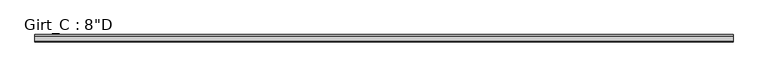
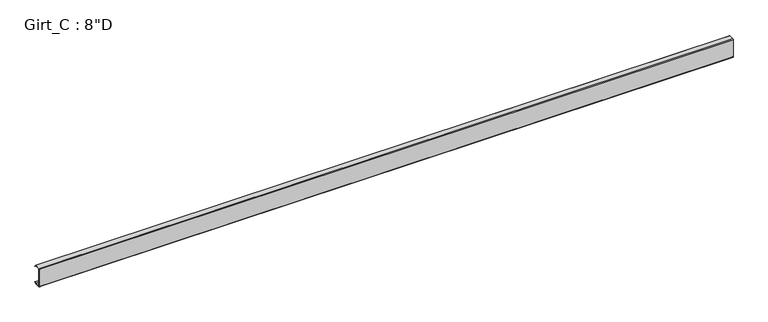
"""IFC4 building model written with IfcOpenShell, lengths in millimetres: beam geometry."""

from ifc_helpers import new_model, si_unit, point, frame, frame_2d, origin, place, context, project, spatial, polyline, circle_curve, trimmed, segment, composite_curve, outline, extrude, source, transform, mapped, element, save


def beam_1497706d(model_context):
    return source(origin(), model_context, "Body", "SweptSolid", [
        extrude(outline(composite_curve([segment(polyline([(63.5, 101.6), (75.745104, 87.0068534), (73.6169367, 85.221109), (62.204539, 98.821875), (3.3005807, 98.821875)]), True, "CONTINUOUS"), segment(trimmed(circle_curve(frame_2d((3.3741066, 96.8381931)), 1.9850441), [point((3.3005807, 98.821875))], [point((1.3890625, 96.8381931))], True, "CARTESIAN"), True, "CONTINUOUS"), segment(polyline([(1.3890625, 96.8381931), (1.3890625, -96.8389339)]), True, "CONTINUOUS"), segment(trimmed(circle_curve(frame_2d((3.3748024, -96.8389339)), 1.9857399), [point((1.3890625, -96.8389339))], [point((3.2694106, -98.821875))], True, "CARTESIAN"), True, "CONTINUOUS"), segment(polyline([(3.2694106, -98.821875), (62.204539, -98.821875), (73.6169367, -85.221109), (75.745104, -87.0068534), (63.5, -101.6), (3.3734375, -101.6)]), True, "CONTINUOUS"), segment(trimmed(circle_curve(frame_2d((3.3734375, -96.8375)), 4.7625), [point((3.3734375, -101.6))], [point((-1.3890625, -96.8375))], False, "CARTESIAN"), True, "CONTINUOUS"), segment(polyline([(-1.3890625, -96.8375), (-1.3890625, 96.8375)]), True, "CONTINUOUS"), segment(trimmed(circle_curve(frame_2d((3.3734375, 96.8375)), 4.7625), [point((-1.3890625, 96.8375))], [point((3.3734375, 101.6))], False, "CARTESIAN"), True, "CONTINUOUS"), segment(polyline([(3.3734375, 101.6), (63.5, 101.6)]), True, "CONTINUOUS")], self_intersect=False)), frame((-3670.3, 0.0, 0.0), z_axis=(1.0, 0.0, 0.0), x_axis=(0.0, 1.0, 0.0)), (0.0, 0.0, 1.0), 7340.6),
    ])


if __name__ == "__main__":
    model = new_model("IFC4")
    model_context = context("Model", 3, world=origin())
    ifc_project = project(units=[si_unit("LENGTHUNIT", "METRE", prefix="MILLI")], contexts=[model_context])
    site = spatial("IfcSite", under=ifc_project)
    building = spatial("IfcBuilding", under=site)
    placement = place(None, origin())
    beam_shape = beam_1497706d(model_context)
    element("IfcBeam", 1, ObjectType="Girt_C : 8\"D", at=placement, inside=building, context=model_context, shape_type="MappedRepresentation", body=[
        mapped(beam_shape, transform((0.0, 0.0, 0.0), x_axis=(1.0, 0.0, 0.0), y_axis=(0.0, 1.0, 0.0), z_axis=(0.0, 0.0, 1.0))),
    ])
    save(model, "model.ifc")

# Revit data of these elements
# Type "Girt_C : 8\"D"
#   Web_Thickness = 0' - 0 7/64"
#   Length [instance default] = 10' - 0"
#   Leg_1 = 0' - 2 1/2"
#   Height = 0' - 8"
#   Structural Material [instance default] = none
# Element 1 (IfcBeam, "Girt_C : 8\"D")
#   Structural Material = Steel
#   Materials on its faces: "Steel"
# Materials
#   "Steel": class "Metal", colour RGB 118 118 114, transparency 0, Description = "Steel, mill finish", Cost = 0
